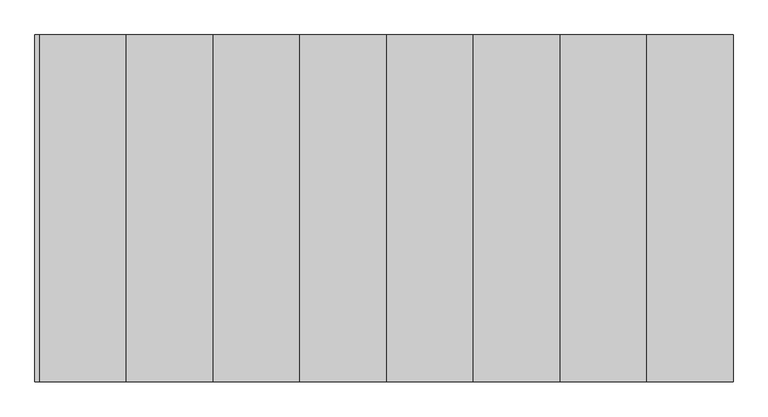
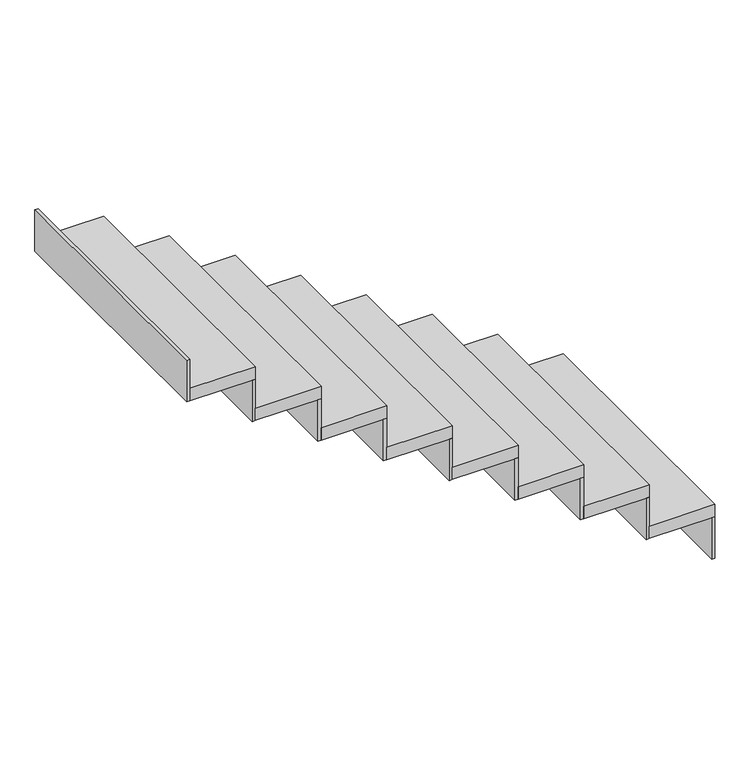
"""IFC4 building model written with IfcOpenShell, lengths in millimetres: stair flight geometry."""

from ifc_helpers import new_model, si_unit, frame, origin, place, context, project, spatial, polyline, outline, extrude, source, transform, mapped, element, save


def stair_flight_f3270307(model_context):
    return source(origin(), model_context, "Body", "SweptSolid", [
        extrude(outline(polyline([(5264.0556606, 2510.81281), (5276.5556606, 2510.81281), (5276.5556606, 1510.81281), (5264.0556606, 1510.81281), (5264.0556606, 2510.81281)])), frame((0.0, 0.0, 4750.0), z_axis=(0.0, 0.0, 1.0), x_axis=(1.0, 0.0, 0.0)), (0.0, 0.0, 1.0), 166.6666667),
        extrude(outline(polyline([(5026.5556606, 1510.81281), (5026.5556606, 2510.81281), (5276.5556606, 2510.81281), (5276.5556606, 1510.81281), (5026.5556606, 1510.81281)])), frame((0.0, 0.0, 4916.6666667), z_axis=(0.0, 0.0, 1.0), x_axis=(1.0, 0.0, 0.0)), (0.0, 0.0, 1.0), 50.0),
        extrude(outline(polyline([(5014.0556606, 2510.81281), (5026.5556606, 2510.81281), (5026.5556606, 1510.81281), (5014.0556606, 1510.81281), (5014.0556606, 2510.81281)])), frame((0.0, 0.0, 4916.6666667), z_axis=(0.0, 0.0, 1.0), x_axis=(1.0, 0.0, 0.0)), (0.0, 0.0, 1.0), 166.6666667),
        extrude(outline(polyline([(4776.5556606, 1510.81281), (4776.5556606, 2510.81281), (5026.5556606, 2510.81281), (5026.5556606, 1510.81281), (4776.5556606, 1510.81281)])), frame((0.0, 0.0, 5083.3333333), z_axis=(0.0, 0.0, 1.0), x_axis=(1.0, 0.0, 0.0)), (0.0, 0.0, 1.0), 50.0),
        extrude(outline(polyline([(4764.0556606, 2510.81281), (4776.5556606, 2510.81281), (4776.5556606, 1510.81281), (4764.0556606, 1510.81281), (4764.0556606, 2510.81281)])), frame((0.0, 0.0, 5083.3333333), z_axis=(0.0, 0.0, 1.0), x_axis=(1.0, 0.0, 0.0)), (0.0, 0.0, 1.0), 166.6666667),
        extrude(outline(polyline([(4526.5556606, 1510.81281), (4526.5556606, 2510.81281), (4776.5556606, 2510.81281), (4776.5556606, 1510.81281), (4526.5556606, 1510.81281)])), frame((0.0, 0.0, 5250.0), z_axis=(0.0, 0.0, 1.0), x_axis=(1.0, 0.0, 0.0)), (0.0, 0.0, 1.0), 50.0),
        extrude(outline(polyline([(4514.0556606, 2510.81281), (4526.5556606, 2510.81281), (4526.5556606, 1510.81281), (4514.0556606, 1510.81281), (4514.0556606, 2510.81281)])), frame((0.0, 0.0, 5250.0), z_axis=(0.0, 0.0, 1.0), x_axis=(1.0, 0.0, 0.0)), (0.0, 0.0, 1.0), 166.6666667),
        extrude(outline(polyline([(4276.5556606, 1510.81281), (4276.5556606, 2510.81281), (4526.5556606, 2510.81281), (4526.5556606, 1510.81281), (4276.5556606, 1510.81281)])), frame((0.0, 0.0, 5416.6666667), z_axis=(0.0, 0.0, 1.0), x_axis=(1.0, 0.0, 0.0)), (0.0, 0.0, 1.0), 50.0),
        extrude(outline(polyline([(4264.0556606, 2510.81281), (4276.5556606, 2510.81281), (4276.5556606, 1510.81281), (4264.0556606, 1510.81281), (4264.0556606, 2510.81281)])), frame((0.0, 0.0, 5416.6666667), z_axis=(0.0, 0.0, 1.0), x_axis=(1.0, 0.0, 0.0)), (0.0, 0.0, 1.0), 166.6666667),
        extrude(outline(polyline([(4026.5556606, 1510.81281), (4026.5556606, 2510.81281), (4276.5556606, 2510.81281), (4276.5556606, 1510.81281), (4026.5556606, 1510.81281)])), frame((0.0, 0.0, 5583.3333333), z_axis=(0.0, 0.0, 1.0), x_axis=(1.0, 0.0, 0.0)), (0.0, 0.0, 1.0), 50.0),
        extrude(outline(polyline([(4014.0556606, 2510.81281), (4026.5556606, 2510.81281), (4026.5556606, 1510.81281), (4014.0556606, 1510.81281), (4014.0556606, 2510.81281)])), frame((0.0, 0.0, 5583.3333333), z_axis=(0.0, 0.0, 1.0), x_axis=(1.0, 0.0, 0.0)), (0.0, 0.0, 1.0), 166.6666667),
        extrude(outline(polyline([(3776.5556606, 1510.81281), (3776.5556606, 2510.81281), (4026.5556606, 2510.81281), (4026.5556606, 1510.81281), (3776.5556606, 1510.81281)])), frame((0.0, 0.0, 5750.0), z_axis=(0.0, 0.0, 1.0), x_axis=(1.0, 0.0, 0.0)), (0.0, 0.0, 1.0), 50.0),
        extrude(outline(polyline([(3764.0556606, 2510.81281), (3776.5556606, 2510.81281), (3776.5556606, 1510.81281), (3764.0556606, 1510.81281), (3764.0556606, 2510.81281)])), frame((0.0, 0.0, 5750.0), z_axis=(0.0, 0.0, 1.0), x_axis=(1.0, 0.0, 0.0)), (0.0, 0.0, 1.0), 166.6666667),
        extrude(outline(polyline([(3526.5556606, 1510.81281), (3526.5556606, 2510.81281), (3776.5556606, 2510.81281), (3776.5556606, 1510.81281), (3526.5556606, 1510.81281)])), frame((0.0, 0.0, 5916.6666667), z_axis=(0.0, 0.0, 1.0), x_axis=(1.0, 0.0, 0.0)), (0.0, 0.0, 1.0), 50.0),
        extrude(outline(polyline([(3514.0556606, 2510.81281), (3526.5556606, 2510.81281), (3526.5556606, 1510.81281), (3514.0556606, 1510.81281), (3514.0556606, 2510.81281)])), frame((0.0, 0.0, 5916.6666667), z_axis=(0.0, 0.0, 1.0), x_axis=(1.0, 0.0, 0.0)), (0.0, 0.0, 1.0), 166.6666667),
        extrude(outline(polyline([(3264.0556606, 2510.81281), (3276.5556606, 2510.81281), (3276.5556606, 1510.81281), (3264.0556606, 1510.81281), (3264.0556606, 2510.81281)])), frame((0.0, 0.0, 6083.3333333), z_axis=(0.0, 0.0, 1.0), x_axis=(1.0, 0.0, 0.0)), (0.0, 0.0, 1.0), 166.6666667),
        extrude(outline(polyline([(3276.5556606, 1510.81281), (3276.5556606, 2510.81281), (3526.5556606, 2510.81281), (3526.5556606, 1510.81281), (3276.5556606, 1510.81281)])), frame((0.0, 0.0, 6083.3333333), z_axis=(0.0, 0.0, 1.0), x_axis=(1.0, 0.0, 0.0)), (0.0, 0.0, 1.0), 50.0),
    ])


if __name__ == "__main__":
    model = new_model("IFC4")
    model_context = context("Model", 3, world=origin())
    ifc_project = project(units=[si_unit("LENGTHUNIT", "METRE", prefix="MILLI")], contexts=[model_context])
    site = spatial("IfcSite", under=ifc_project)
    building = spatial("IfcBuilding", under=site)
    placement = place(None, origin())
    stair_flight_shape = stair_flight_f3270307(model_context)
    element("IfcStairFlight", 1, at=placement, inside=building, context=model_context, shape_type="MappedRepresentation", body=[
        mapped(stair_flight_shape, transform((0.0, 0.0, 0.0), x_axis=(1.0, 0.0, 0.0), y_axis=(0.0, 1.0, 0.0), z_axis=(0.0, 0.0, 1.0))),
    ])
    save(model, "model.ifc")
